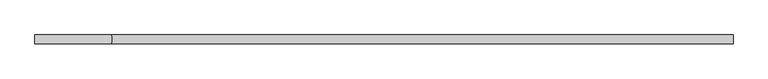
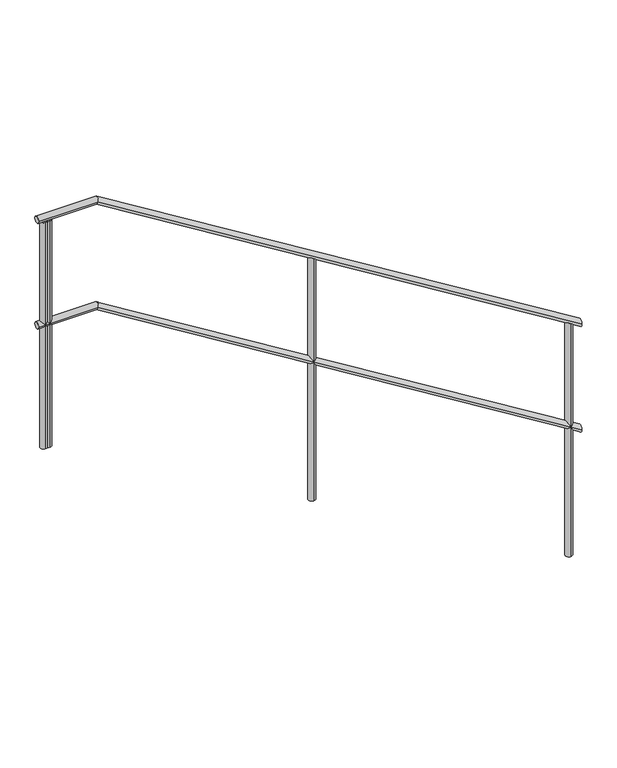
"""IFC4 building model written with IfcOpenShell, lengths in millimetres: railing geometry."""

from ifc_helpers import new_model, si_unit, point, frame, frame_2d, origin, place, context, project, spatial, circle_curve, ellipse_curve, trimmed, segment, composite_curve, outline, extrude, source, transform, mapped, element, save
from ifc_brep_helpers import plane_surface, cylinder_surface, advanced_brep


def railing_d00e91c8(model_context):
    return source(origin(), model_context, "Body", "SolidModel", [
        advanced_brep(
        [(33992.1378478, 63512.0208589, -450.9609787), (33992.1378478, 63542.0208589, -450.9609787), (31827.8810623, 63512.0208589, 885.0), (31827.8810623, 63542.0208589, 885.0), (31562.1378478, 63512.0208589, 885.0), (31562.1378478, 63542.0208589, 885.0)],
        [
            (0, 1, ellipse_curve(frame((33992.1378478, 63527.0208589, -450.9609787), z_axis=(1.0, 0.0, 0.0), x_axis=(0.0, 0.0, -1.0)), 17.6276454, 15.0)),
            (1, 0, ellipse_curve(frame((33992.1378478, 63527.0208589, -450.9609787), z_axis=(1.0, 0.0, 0.0), x_axis=(0.0, 0.0, -1.0)), 17.6276454, 15.0)),
            (0, 2),
            (2, 3, ellipse_curve(frame((31827.8810623, 63527.0208589, 885.0), z_axis=(0.9620125025549408, 0.0, -0.2730053935877092), x_axis=(-0.2730053935877086, 0.0, -0.9620125025549411)), 15.5923129, 15.0)),
            (3, 1),
            (3, 2, ellipse_curve(frame((31827.8810623, 63527.0208589, 885.0), z_axis=(0.9620125025549408, 0.0, -0.2730053935877092), x_axis=(-0.2730053935877086, 0.0, -0.9620125025549411)), 15.5923129, 15.0)),
            (4, 5, circle_curve(frame((31562.1378478, 63527.0208589, 885.0), z_axis=(-1.0, 0.0, 0.0), x_axis=(0.0, 1.0, 0.0)), 15.0)),
            (5, 4, circle_curve(frame((31562.1378478, 63527.0208589, 885.0), z_axis=(-1.0, 0.0, 0.0), x_axis=(0.0, 1.0, 0.0)), 15.0)),
            (2, 4),
            (5, 3),
        ],
        [
            plane_surface(frame((33992.1378478, 63527.0208589, -433.3333333), z_axis=(1.0, 0.0, 0.0), x_axis=(0.0, -1.0, 0.0))),
            cylinder_surface(frame((33984.2588097, 63527.0208589, -446.097375), z_axis=(0.8509361101440399, 0.0, -0.5252692037926175), x_axis=(0.0, 1.0, 0.0)), 15.0),
            plane_surface(frame((31562.1378478, 63527.0208589, 900.0), z_axis=(-1.0, 0.0, 0.0), x_axis=(0.0, -1.0, 0.0))),
            cylinder_surface(frame((31832.1378478, 63527.0208589, 885.0), z_axis=(1.0, 0.0, 0.0), x_axis=(0.0, 1.0, 0.0)), 15.0),
        ],
        [
            (0, [[1, 2]]),
            (1, [[-1, 3, 4, 5]]),
            (1, [[-2, -5, 6, -3]]),
            (2, [[7, 8]]),
            (3, [[-4, 9, -8, 10]]),
            (3, [[-6, -10, -7, -9]]),
        ],
    ),
        advanced_brep(
        [(33992.1378478, 63512.0208589, 49.0390213), (33992.1378478, 63542.0208589, 49.0390213), (31827.8810623, 63512.0208589, 1385.0), (31827.8810623, 63542.0208589, 1385.0), (31562.1378478, 63512.0208589, 1385.0), (31562.1378478, 63542.0208589, 1385.0)],
        [
            (0, 1, ellipse_curve(frame((33992.1378478, 63527.0208589, 49.0390213), z_axis=(1.0, 0.0, 0.0), x_axis=(0.0, 0.0, -1.0)), 17.6276454, 15.0)),
            (1, 0, ellipse_curve(frame((33992.1378478, 63527.0208589, 49.0390213), z_axis=(1.0, 0.0, 0.0), x_axis=(0.0, 0.0, -1.0)), 17.6276454, 15.0)),
            (0, 2),
            (2, 3, ellipse_curve(frame((31827.8810623, 63527.0208589, 1385.0), z_axis=(0.9620125025549408, 0.0, -0.2730053935877092), x_axis=(-0.2730053935877086, 0.0, -0.9620125025549411)), 15.5923129, 15.0)),
            (3, 1),
            (3, 2, ellipse_curve(frame((31827.8810623, 63527.0208589, 1385.0), z_axis=(0.9620125025549408, 0.0, -0.2730053935877092), x_axis=(-0.2730053935877086, 0.0, -0.9620125025549411)), 15.5923129, 15.0)),
            (4, 5, circle_curve(frame((31562.1378478, 63527.0208589, 1385.0), z_axis=(-1.0, 0.0, 0.0), x_axis=(0.0, 1.0, 0.0)), 15.0)),
            (5, 4, circle_curve(frame((31562.1378478, 63527.0208589, 1385.0), z_axis=(-1.0, 0.0, 0.0), x_axis=(0.0, 1.0, 0.0)), 15.0)),
            (2, 4),
            (5, 3),
        ],
        [
            plane_surface(frame((33992.1378478, 63527.0208589, 66.6666667), z_axis=(1.0, 0.0, 0.0), x_axis=(0.0, -1.0, 0.0))),
            cylinder_surface(frame((33984.2588097, 63527.0208589, 53.902625), z_axis=(0.8509361101440399, 0.0, -0.5252692037926175), x_axis=(0.0, 1.0, 0.0)), 15.0),
            plane_surface(frame((31562.1378478, 63527.0208589, 1400.0), z_axis=(-1.0, 0.0, 0.0), x_axis=(0.0, -1.0, 0.0))),
            cylinder_surface(frame((31832.1378478, 63527.0208589, 1385.0), z_axis=(1.0, 0.0, 0.0), x_axis=(0.0, 1.0, 0.0)), 15.0),
        ],
        [
            (0, [[1, 2]]),
            (1, [[-1, 3, 4, 5]]),
            (1, [[-2, -5, 6, -3]]),
            (2, [[7, 8]]),
            (3, [[-4, 9, -8, 10]]),
            (3, [[-6, -10, -7, -9]]),
        ],
    ),
        extrude(outline(composite_curve([segment(trimmed(circle_curve(frame_2d((31592.1378478, 63527.0208589)), 15.0), [point((31592.1378478, 63512.0208589))], [point((31592.1378478, 63542.0208589))], False, "CARTESIAN"), True, "CONTINUOUS"), segment(trimmed(circle_curve(frame_2d((31592.1378478, 63527.0208589)), 15.0), [point((31592.1378478, 63542.0208589))], [point((31592.1378478, 63512.0208589))], False, "CARTESIAN"), True, "CONTINUOUS")], self_intersect=False)), frame((0.0, 0.0, 300.0), z_axis=(0.0, 0.0, 1.0), x_axis=(1.0, 0.0, 0.0)), (0.0, 0.0, 1.0), 1070.0),
        advanced_brep(
        [(32792.1378478, 63542.0208589, 777.4074074), (32792.1378478, 63542.0208589, -366.6666667), (32792.1378478, 63512.0208589, -366.6666667), (32792.1378478, 63512.0208589, 777.4074074)],
        [
            (0, 1),
            (1, 2, circle_curve(frame((32792.1378478, 63527.0208589, -366.6666667), z_axis=(0.0, 0.0, 1.0), x_axis=(0.0, -1.0, 0.0)), 15.0)),
            (2, 3),
            (3, 0, ellipse_curve(frame((32792.1378478, 63527.0208589, 777.4074074), z_axis=(-0.5252692037926167, 0.0, -0.8509361101440406), x_axis=(-0.8509361101440406, 0.0, 0.5252692037926162)), 17.6276454, 15.0)),
            (0, 3, ellipse_curve(frame((32792.1378478, 63527.0208589, 777.4074074), z_axis=(-0.5252692037926167, 0.0, -0.8509361101440406), x_axis=(-0.8509361101440406, 0.0, 0.5252692037926162)), 17.6276454, 15.0)),
            (2, 1, circle_curve(frame((32792.1378478, 63527.0208589, -366.6666667), z_axis=(0.0, 0.0, 1.0), x_axis=(0.0, -1.0, 0.0)), 15.0)),
        ],
        [
            cylinder_surface(frame((32792.1378478, 63527.0208589, -466.6666667), z_axis=(0.0, 0.0, 1.0), x_axis=(0.0, -1.0, 0.0)), 15.0),
            plane_surface(frame((32767.1378478, 63502.0208589, 792.8395062), z_axis=(0.5252692037926167, 0.0, 0.8509361101440406), x_axis=(0.0, 1.0, 0.0))),
            plane_surface(frame((32817.1378478, 63502.0208589, -366.6666667), z_axis=(0.0, 0.0, -1.0), x_axis=(0.0, 1.0, 0.0))),
        ],
        [
            (0, [[1, 2, 3, 4]]),
            (0, [[-1, 5, -3, 6]]),
            (1, [[-4, -5]]),
            (2, [[-2, -6]]),
        ],
    ),
        extrude(outline(composite_curve([segment(trimmed(circle_curve(frame_2d((31612.1378478, 63527.0208589)), 15.0), [point((31612.1378478, 63512.0208589))], [point((31612.1378478, 63542.0208589))], False, "CARTESIAN"), True, "CONTINUOUS"), segment(trimmed(circle_curve(frame_2d((31612.1378478, 63527.0208589)), 15.0), [point((31612.1378478, 63542.0208589))], [point((31612.1378478, 63512.0208589))], False, "CARTESIAN"), True, "CONTINUOUS")], self_intersect=False)), frame((0.0, 0.0, 300.0), z_axis=(0.0, 0.0, 1.0), x_axis=(1.0, 0.0, 0.0)), (0.0, 0.0, 1.0), 1070.0),
        advanced_brep(
        [(33942.1378478, 63542.0208589, 67.5308642), (33942.1378478, 63542.0208589, -1033.3333333), (33942.1378478, 63512.0208589, -1033.3333333), (33942.1378478, 63512.0208589, 67.5308642)],
        [
            (0, 1),
            (1, 2, circle_curve(frame((33942.1378478, 63527.0208589, -1033.3333333), z_axis=(0.0, 0.0, 1.0), x_axis=(0.0, -1.0, 0.0)), 15.0)),
            (2, 3),
            (3, 0, ellipse_curve(frame((33942.1378478, 63527.0208589, 67.5308642), z_axis=(-0.5252692037926167, 0.0, -0.8509361101440406), x_axis=(-0.8509361101440406, 0.0, 0.5252692037926162)), 17.6276454, 15.0)),
            (0, 3, ellipse_curve(frame((33942.1378478, 63527.0208589, 67.5308642), z_axis=(-0.5252692037926167, 0.0, -0.8509361101440406), x_axis=(-0.8509361101440406, 0.0, 0.5252692037926162)), 17.6276454, 15.0)),
            (2, 1, circle_curve(frame((33942.1378478, 63527.0208589, -1033.3333333), z_axis=(0.0, 0.0, 1.0), x_axis=(0.0, -1.0, 0.0)), 15.0)),
        ],
        [
            cylinder_surface(frame((33942.1378478, 63527.0208589, -1133.3333333), z_axis=(0.0, 0.0, 1.0), x_axis=(0.0, -1.0, 0.0)), 15.0),
            plane_surface(frame((33917.1378478, 63502.0208589, 82.962963), z_axis=(0.5252692037926167, 0.0, 0.8509361101440406), x_axis=(0.0, 1.0, 0.0))),
            plane_surface(frame((33967.1378478, 63502.0208589, -1033.3333333), z_axis=(0.0, 0.0, -1.0), x_axis=(0.0, 1.0, 0.0))),
        ],
        [
            (0, [[1, 2, 3, 4]]),
            (0, [[-1, 5, -3, 6]]),
            (1, [[-4, -5]]),
            (2, [[-2, -6]]),
        ],
    ),
    ])


if __name__ == "__main__":
    model = new_model("IFC4")
    model_context = context("Model", 3, world=origin())
    ifc_project = project(units=[si_unit("LENGTHUNIT", "METRE", prefix="MILLI")], contexts=[model_context])
    site = spatial("IfcSite", under=ifc_project)
    building = spatial("IfcBuilding", under=site)
    placement = place(None, origin())
    railing_shape = railing_d00e91c8(model_context)
    element("IfcRailing", 1, at=placement, inside=building, context=model_context, shape_type="MappedRepresentation", body=[
        mapped(railing_shape, transform((0.0, 0.0, 0.0), x_axis=(1.0, 0.0, 0.0), y_axis=(0.0, 1.0, 0.0), z_axis=(0.0, 0.0, 1.0))),
    ])
    save(model, "model.ifc")
